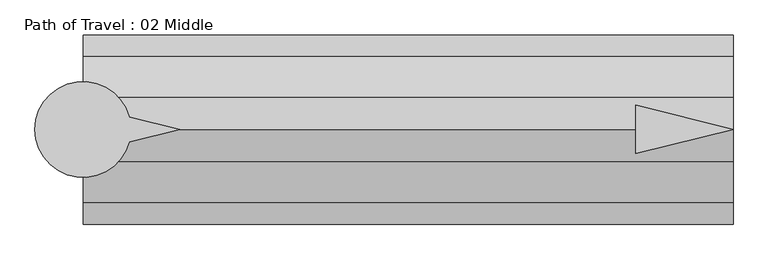
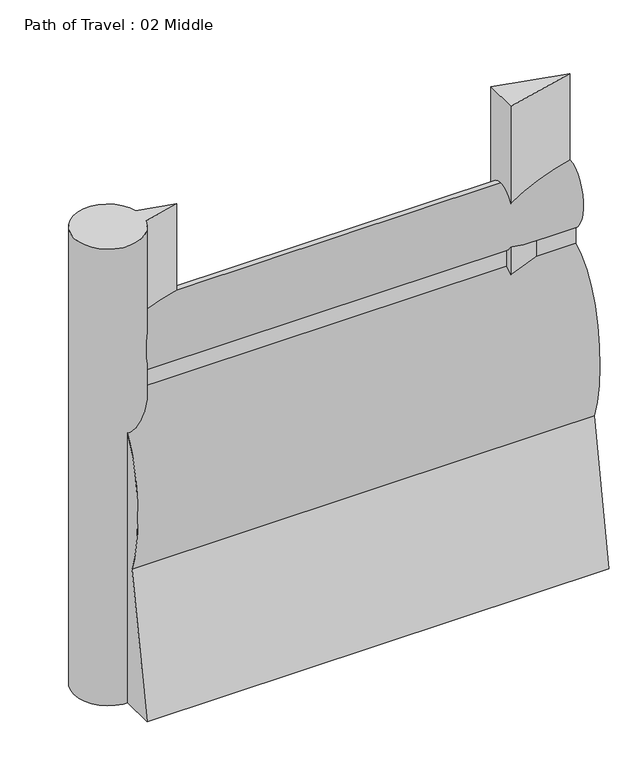
"""IFC4 building model written with IfcOpenShell, lengths in millimetres: proxy geometry, Path of Travel : 02 Middle."""

from ifc_helpers import new_model, si_unit, point, frame, frame_2d, origin, origin_with_axes, place, context, project, spatial, polyline, circle_curve, ellipse_curve, trimmed, segment, composite_curve, outline, extrude, source, transform, mapped, element, save
from ifc_brep_helpers import plane_surface, extruded_surface, advanced_brep


def path_of_travel_02_middle_ae4c9040(model_context):
    return source(origin(), model_context, "Body", "SolidModel", [
        advanced_brep(
        [(227.5554837, 0.0, 1727.2), (227.5554837, 42.9018657, 1436.6534209), (227.5554837, 42.9018657, 1363.4763406), (227.5554837, 184.1186263, 643.4144547), (227.5554837, 297.5699544, 0.0), (227.5554837, 145.6574193, 0.0), (227.5554837, 0.0, 584.2), (227.5554837, -145.6574193, 0.0), (227.5554837, -297.5699544, 0.0), (227.5554837, -184.1186263, 643.4144547), (227.5554837, -42.9018657, 1363.4763406), (227.5554837, -42.9018657, 1436.6534209), (2268.4123179, 0.0, 1727.2), (2268.4123179, -42.9018657, 1436.6534209), (2268.4123179, -42.9018657, 1363.4763406), (2268.4123179, -184.1186263, 643.4144547), (2268.4123179, -297.5699544, 0.0), (2268.4123179, -145.6574193, 0.0), (2268.4123179, 0.0, 584.2), (2268.4123179, 145.6574193, 0.0), (2268.4123179, 297.5699544, 0.0), (2268.4123179, 184.1186263, 643.4144547), (2268.4123179, 42.9018657, 1363.4763406), (2268.4123179, 42.9018657, 1436.6534209)],
        [
            (0, 1, ellipse_curve(frame((227.5554837, 0.0, 1574.8), z_axis=(-1.0, 0.0, 0.0), x_axis=(0.0, 0.0, 1.0)), 152.4, 101.6)),
            (1, 2),
            (2, 3, ellipse_curve(frame((227.5554837, 0.0, 914.4), z_axis=(-1.0, 0.0, 0.0), x_axis=(0.0, 0.0, -1.0)), 457.2, 228.6)),
            (3, 4),
            (4, 5),
            (5, 6),
            (6, 7),
            (7, 8),
            (8, 9),
            (9, 10, ellipse_curve(frame((227.5554837, 0.0, 914.4), z_axis=(-1.0, 0.0, 0.0), x_axis=(0.0, 0.0, -1.0)), 457.2, 228.6)),
            (10, 11),
            (11, 0, ellipse_curve(frame((227.5554837, 0.0, 1574.8), z_axis=(-1.0, 0.0, 0.0), x_axis=(0.0, 0.0, 1.0)), 152.4, 101.6)),
            (12, 13, ellipse_curve(frame((2268.4123179, 0.0, 1574.8), z_axis=(1.0, 0.0, 0.0), x_axis=(0.0, 0.0, 1.0)), 152.4, 101.6)),
            (13, 14),
            (14, 15, ellipse_curve(frame((2268.4123179, 0.0, 914.4), z_axis=(1.0, 0.0, 0.0), x_axis=(0.0, 0.0, -1.0)), 457.2, 228.6)),
            (15, 16),
            (16, 17),
            (17, 18),
            (18, 19),
            (19, 20),
            (20, 21),
            (21, 22, ellipse_curve(frame((2268.4123179, 0.0, 914.4), z_axis=(1.0, 0.0, 0.0), x_axis=(0.0, 0.0, -1.0)), 457.2, 228.6)),
            (22, 23),
            (23, 12, ellipse_curve(frame((2268.4123179, 0.0, 1574.8), z_axis=(1.0, 0.0, 0.0), x_axis=(0.0, 0.0, 1.0)), 152.4, 101.6)),
            (0, 12),
            (23, 1),
            (22, 2),
            (21, 3),
            (20, 4),
            (19, 5),
            (18, 6),
            (17, 7),
            (16, 8),
            (15, 9),
            (14, 10),
            (13, 11),
        ],
        [
            plane_surface(frame((227.5554837, 0.0, 0.0), z_axis=(-1.0, 0.0, 0.0), x_axis=(0.0, 0.0, 1.0))),
            plane_surface(frame((2268.4123179, 0.0, 0.0), z_axis=(1.0, 0.0, 0.0), x_axis=(0.0, 0.0, 1.0))),
            extruded_surface(trimmed(ellipse_curve(frame((2268.4123179, 0.0, 1574.8), z_axis=(-1.0, 0.0, 0.0), x_axis=(0.0, 0.0, 1.0)), 152.4, 101.6), [point((2268.4123179, 0.0, 1727.2))], [point((2268.4123179, 42.9018657, 1436.6534209))], True, "CARTESIAN"), (-2040.8568341999999, 0.0, 0.0), 2040.8568341999999),
            plane_surface(frame((227.5554837, 42.9018657, 1436.6534209), z_axis=(0.0, 1.0, 0.0), x_axis=(1.0, 0.0, 0.0))),
            extruded_surface(trimmed(ellipse_curve(frame((2268.4123179, 0.0, 914.4), z_axis=(-1.0, 0.0, 0.0), x_axis=(0.0, 0.0, -1.0)), 457.2, 228.6), [point((2268.4123179, 42.9018657, 1363.4763406))], [point((2268.4123179, 184.1186263, 643.4144547))], True, "CARTESIAN"), (-2040.8568341999999, 0.0, 0.0), 2040.8568341999999),
            plane_surface(frame((227.5554837, 184.1186263, 643.4144547), z_axis=(0.0, 0.9848077530122078, 0.1736481776669322), x_axis=(1.0, 0.0, 0.0))),
            plane_surface(frame((227.5554837, 297.5699544, 0.0), z_axis=(0.0, 0.0, -1.0), x_axis=(1.0, 0.0, 0.0))),
            plane_surface(frame((227.5554837, 145.6574193, 0.0), z_axis=(0.0, -0.9702957262760199, -0.2419218955995739), x_axis=(1.0, 0.0, 0.0))),
            plane_surface(frame((227.5554837, 0.0, 584.2), z_axis=(0.0, 0.9702957262759961, -0.24192189559966923), x_axis=(1.0, 0.0, 0.0))),
            plane_surface(frame((227.5554837, -145.6574193, 0.0), z_axis=(0.0, 0.0, -1.0), x_axis=(1.0, 0.0, 0.0))),
            plane_surface(frame((227.5554837, -297.5699544, 0.0), z_axis=(0.0, -0.984807753012208, 0.17364817766693066), x_axis=(1.0, 0.0, 0.0))),
            extruded_surface(trimmed(ellipse_curve(frame((2268.4123179, 0.0, 914.4), z_axis=(-1.0, 0.0, 0.0), x_axis=(0.0, 0.0, -1.0)), 457.2, 228.6), [point((2268.4123179, -184.1186263, 643.4144547))], [point((2268.4123179, -42.9018657, 1363.4763406))], True, "CARTESIAN"), (-2040.8568341999999, 0.0, 0.0), 2040.8568341999999),
            plane_surface(frame((227.5554837, -42.9018657, 1363.4763406), z_axis=(0.0, -1.0, 0.0), x_axis=(1.0, 0.0, 0.0))),
            extruded_surface(trimmed(ellipse_curve(frame((2268.4123179, 0.0, 1574.8), z_axis=(-1.0, 0.0, 0.0), x_axis=(0.0, 0.0, 1.0)), 152.4, 101.6), [point((2268.4123179, -42.9018657, 1436.6534209))], [point((2268.4123179, 0.0, 1727.2))], True, "CARTESIAN"), (-2040.8568341999999, 0.0, 0.0), 2040.8568341999999),
        ],
        [
            (0, [[1, 2, 3, 4, 5, 6, 7, 8, 9, 10, 11, 12]]),
            (1, [[13, 14, 15, 16, 17, 18, 19, 20, 21, 22, 23, 24]]),
            (2, [[-1, 25, -24, 26]]),
            (3, [[-2, -26, -23, 27]]),
            (4, [[-3, -27, -22, 28]]),
            (5, [[-4, -28, -21, 29]]),
            (6, [[-5, -29, -20, 30]]),
            (7, [[-6, -30, -19, 31]]),
            (8, [[-7, -31, -18, 32]]),
            (9, [[-8, -32, -17, 33]]),
            (10, [[-9, -33, -16, 34]]),
            (11, [[-10, -34, -15, 35]]),
            (12, [[-11, -35, -14, 36]]),
            (13, [[-12, -36, -13, -25]]),
        ],
    ),
        extrude(outline(polyline([(1962.4071713, 76.2006338), (2268.4123179, 0.0), (1962.4071713, -76.2006338), (1962.4071713, 76.2006338)])), origin_with_axes(), (0.0, 0.0, 1.0), 2129.5973753),
        extrude(outline(composite_curve([segment(polyline([(372.7837828, 39.4440225), (531.182385, 0.0), (372.7837828, -39.4440225)]), True, "CONTINUOUS"), segment(trimmed(circle_curve(frame_2d((227.2200886, 0.0)), 150.8131956), [point((372.7837828, -39.4440225))], [point((372.7837828, 39.4440225))], False, "CARTESIAN"), True, "CONTINUOUS")], self_intersect=False)), origin_with_axes(), (0.0, 0.0, 1.0), 2129.5973753),
    ])


if __name__ == "__main__":
    model = new_model("IFC4")
    model_context = context("Model", 3, world=origin())
    ifc_project = project(units=[si_unit("LENGTHUNIT", "METRE", prefix="MILLI")], contexts=[model_context])
    site = spatial("IfcSite", under=ifc_project)
    building = spatial("IfcBuilding", under=site)
    placement = place(None, origin())
    path_of_travel_02_middle_shape = path_of_travel_02_middle_ae4c9040(model_context)
    element("IfcBuildingElementProxy", 1, Name="Path of Travel : 02 Middle", ObjectType="Path of Travel : 02 Middle", at=placement, inside=building, context=model_context, shape_type="MappedRepresentation", body=[
        mapped(path_of_travel_02_middle_shape, transform((0.0, 0.0, 0.0), x_axis=(1.0, 0.0, 0.0), y_axis=(0.0, 1.0, 0.0), z_axis=(0.0, 0.0, 1.0))),
    ])
    save(model, "model.ifc")

# Revit data of these elements
# Type "Path of Travel : 02 Middle"
#   Path of Egress [instance default] = 4' - 0"
#   built-in parameter 1001306 [instance default] = 4 (stored number, unit not read)
#   Dot at Start = no
#   Arrow in Middle = yes
#   Arrow at End = no
#   Egress Path = none
# Element 1 (IfcBuildingElementProxy, "Path of Travel : 02 Middle")
#   Path of Egress = 6' - 8.34869"
#   built-in parameter 1001306 = 6.69572 (stored number, unit not read)
#   Materials on its faces: "Egress Path Solid", "solid"
# Materials
#   "Egress Path Solid": class "Unassigned", colour RGB 255 128 64, transparency 0.75, Comments = "Rendering appearance not upgraded "
#   "solid": class "Generic", colour RGB 120 120 120, transparency 0, Cost = 0
